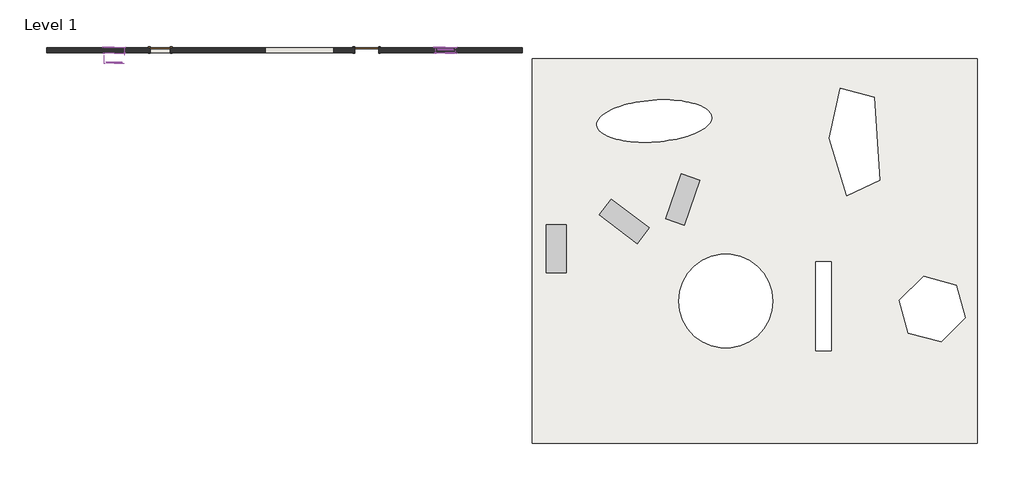
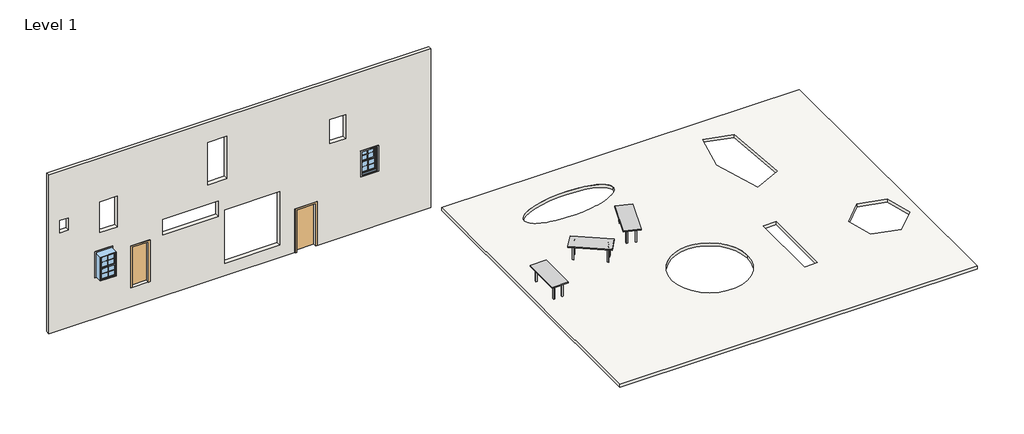
# One storey: 8 proxies, 3 furniture elements, 2 doors, 2 windows, 1 slab, 1 wall.
"""IFC4 building model written with IfcOpenShell, lengths in millimetres."""

import ifcopenshell
import ifcopenshell.guid

model = None  # the IFC model being written
_history = None  # IfcOwnerHistory: only IFC2X3 demands one
_inside = {}  # id of a spatial element -> (the spatial element, [elements in it])
_under = {}  # id of a project, library or spatial element -> (it, [spatial elements below it])
_declared = {}  # id of a project -> (the project, [libraries it declares])
_typed = {}  # id of a type object -> (the type object, [elements of that type])
_made_of = {}  # id of a material, layer set ... -> (it, [elements and type objects made of it])


def new_model(schema):
    """Start an empty IFC model of exactly this schema.

    Asked for "IFC4X3", IfcOpenShell would pick the latest addendum, in which some entities
    have other attributes; the version numbers below select the first issue.
    IFC2X3 requires an IfcOwnerHistory on every rooted entity: one is made here for all.
    """
    global model, _history
    if schema == "IFC4X3":
        model = ifcopenshell.file(schema_version=(4, 3, 0, 0))
    else:
        model = ifcopenshell.file(schema=schema)
    _inside.clear()
    _under.clear()
    _declared.clear()
    _typed.clear()
    _made_of.clear()
    _history = None
    if model.schema == "IFC2X3":
        org = make("IfcOrganization", Name="unknown")
        user = make(
            "IfcPersonAndOrganization",
            ThePerson=make("IfcPerson", FamilyName="unknown"),
            TheOrganization=org,
        )
        app = make(
            "IfcApplication",
            ApplicationDeveloper=org,
            Version="unknown",
            ApplicationFullName="unknown",
            ApplicationIdentifier="unknown",
        )
        _history = make(
            "IfcOwnerHistory",
            OwningUser=user,
            OwningApplication=app,
            ChangeAction="ADDED",
            CreationDate=0,
        )
    return model


def make(cls, **values):
    """One entity of the class cls with the attributes given. An attribute that is None is left unset."""
    return model.create_entity(
        cls, **{name: value for name, value in values.items() if value is not None}
    )


def rooted(cls, **values):
    """An entity with a GlobalId (a new one), such as an element, a storey or a relation."""
    return make(cls, GlobalId=ifcopenshell.guid.new(), OwnerHistory=_history, **values)


def si_unit(unit_type, name, prefix=None):
    """IfcSIUnit, for example si_unit("LENGTHUNIT", "METRE", prefix="MILLI")."""
    return make("IfcSIUnit", UnitType=unit_type, Prefix=prefix, Name=name)


def assignment(units):
    """IfcUnitAssignment: the units of a project."""
    return None if units is None else make("IfcUnitAssignment", Units=units)


def point(xyz):
    """IfcCartesianPoint."""
    return None if xyz is None else make("IfcCartesianPoint", Coordinates=xyz)


def direction(xyz):
    """IfcDirection."""
    return None if xyz is None else make("IfcDirection", DirectionRatios=xyz)


def frame(location, z_axis=None, x_axis=None):
    """IfcAxis2Placement3D, a coordinate frame: its origin and axes. An axis left out is left unset."""
    return make(
        "IfcAxis2Placement3D",
        Location=point(location),
        Axis=direction(z_axis),
        RefDirection=direction(x_axis),
    )


def origin():
    """The frame at (0, 0, 0) with its axes left unset."""
    return frame((0.0, 0.0, 0.0))


def origin_with_axes():
    """The frame at (0, 0, 0) with the z axis (0, 0, 1) and the x axis (1, 0, 0) written out."""
    return frame((0.0, 0.0, 0.0), z_axis=(0.0, 0.0, 1.0), x_axis=(1.0, 0.0, 0.0))


def place(relative_to, where):
    """IfcLocalPlacement: puts the frame where relative to a parent placement (None: the world)."""
    return make(
        "IfcLocalPlacement", PlacementRelTo=relative_to, RelativePlacement=where
    )


def context(
    kind, dimensions, precision=None, world=None, true_north=None, identifier=None
):
    """IfcGeometricRepresentationContext, for example the 3D "Model" context."""
    return make(
        "IfcGeometricRepresentationContext",
        ContextIdentifier=identifier,
        ContextType=kind,
        CoordinateSpaceDimension=dimensions,
        Precision=precision,
        WorldCoordinateSystem=world,
        TrueNorth=true_north,
    )


def project(units=None, contexts=None):
    """IfcProject with its units and contexts."""
    return rooted(
        "IfcProject",
        Name="project",
        RepresentationContexts=contexts,
        UnitsInContext=assignment(units),
    )


def spatial(cls, under=None, at=None, **own):
    """A site, building, storey or space (cls), placed at a placement, below another one or the project."""
    s = rooted(cls, ObjectPlacement=at, **own)
    if under is not None:
        _under.setdefault(under.id(), (under, []))[1].append(s)
    return s


def polyline(points):
    """IfcPolyline through the points."""
    return make("IfcPolyline", Points=[point(p) for p in points])


def circle_curve(where, radius):
    """IfcCircle in the frame where."""
    return make("IfcCircle", Position=where, Radius=radius)


def ellipse_curve(where, semi_axis1, semi_axis2):
    """IfcEllipse in the frame where."""
    return make(
        "IfcEllipse", Position=where, SemiAxis1=semi_axis1, SemiAxis2=semi_axis2
    )


def trimmed(basis, trim1, trim2, sense, master):
    """IfcTrimmedCurve: the piece of a basis curve between two trims."""
    return make(
        "IfcTrimmedCurve",
        BasisCurve=basis,
        Trim1=trim1,
        Trim2=trim2,
        SenseAgreement=sense,
        MasterRepresentation=master,
    )


def outline(outer, holes=None, kind="AREA"):
    """IfcArbitraryClosedProfileDef: a profile drawn as a closed curve; with holes, ...WithVoids."""
    if holes is None:
        return make("IfcArbitraryClosedProfileDef", ProfileType=kind, OuterCurve=outer)
    return make(
        "IfcArbitraryProfileDefWithVoids",
        ProfileType=kind,
        OuterCurve=outer,
        InnerCurves=holes,
    )


def extrude(swept, where, along, depth):
    """IfcExtrudedAreaSolid: the profile swept, set in the frame where, extruded along a direction by depth."""
    return make(
        "IfcExtrudedAreaSolid",
        SweptArea=swept,
        Position=where,
        ExtrudedDirection=direction(along),
        Depth=depth,
    )


def shape(context_of_items, identifier, shape_type, items):
    """IfcShapeRepresentation: the items that make up one representation, for example the "Body"."""
    return make(
        "IfcShapeRepresentation",
        ContextOfItems=context_of_items,
        RepresentationIdentifier=identifier,
        RepresentationType=shape_type,
        Items=items,
    )


def source(mapping_origin, context_of_items, identifier, shape_type, items):
    """IfcRepresentationMap: a shape defined once, which mapped items show again and again."""
    return make(
        "IfcRepresentationMap",
        MappingOrigin=mapping_origin,
        MappedRepresentation=shape(context_of_items, identifier, shape_type, items),
    )


def transform(
    local_origin,
    x_axis=None,
    y_axis=None,
    z_axis=None,
    scale=None,
    scale2=None,
    scale3=None,
    uniform=True,
):
    """IfcCartesianTransformationOperator3D, or its non-uniform kind. x_axis, y_axis, z_axis: its Axis1, 2, 3."""
    if uniform:
        return make(
            "IfcCartesianTransformationOperator3D",
            Axis1=direction(x_axis),
            Axis2=direction(y_axis),
            LocalOrigin=point(local_origin),
            Scale=scale,
            Axis3=direction(z_axis),
        )
    return make(
        "IfcCartesianTransformationOperator3DnonUniform",
        Axis1=direction(x_axis),
        Axis2=direction(y_axis),
        LocalOrigin=point(local_origin),
        Scale=scale,
        Axis3=direction(z_axis),
        Scale2=scale2,
        Scale3=scale3,
    )


def mapped(mapping_source, mapping_target):
    """IfcMappedItem: shows the shape of a source again, moved by a transform."""
    return make(
        "IfcMappedItem", MappingSource=mapping_source, MappingTarget=mapping_target
    )


def made_of(thing, what):
    """Note that an element or type object is made of a material, layer set ...; save() writes the relation."""
    if what is not None:
        _made_of.setdefault(what.id(), (what, []))[1].append(thing)
    return thing


def element(
    cls,
    number,
    at=None,
    inside=None,
    cuts=None,
    type_object=None,
    material=None,
    context=None,
    identifier="Body",
    shape_type=None,
    held_by="IfcProductDefinitionShape",
    body=None,
    shapes=None,
    **own,
):
    """One element of the class cls, such as IfcWall. Its Tag is "e" and its number.

    at: its placement. inside: the storey or other place that contains it. cuts: it is an
    opening in that element (IfcRelVoidsElement). A single representation is given by context,
    identifier, shape_type and body (its items); several are given by shapes. held_by: the class
    of the entity that holds the representations. save() writes the other relations.
    """
    e = rooted(cls, Tag="e%d" % number, ObjectPlacement=at, **own)
    if body is not None:
        shapes = [shape(context, identifier, shape_type, body)]
    if shapes is not None:
        e.Representation = make(held_by, Representations=shapes)
    if inside is not None:
        _inside.setdefault(inside.id(), (inside, []))[1].append(e)
    if cuts is not None:
        rooted(
            "IfcRelVoidsElement", RelatingBuildingElement=cuts, RelatedOpeningElement=e
        )
    if type_object is not None:
        _typed.setdefault(type_object.id(), (type_object, []))[1].append(e)
    return made_of(e, material)


def aggregate(whole, parts):
    """IfcRelAggregates: a whole, such as a stair, and the parts it consists of."""
    return rooted("IfcRelAggregates", RelatingObject=whole, RelatedObjects=parts)


def save(model, path):
    """Write the relations noted so far, then the file.

    IfcRelAggregates (storeys below a building ...), IfcRelContainedInSpatialStructure (elements
    in a storey), IfcRelDefinesByType, IfcRelAssociatesMaterial and IfcRelDeclares: one each for
    every whole, place, type object, material and project.
    """
    for whole, parts in _under.values():
        aggregate(whole, parts)
    for where, things in _inside.values():
        rooted(
            "IfcRelContainedInSpatialStructure",
            RelatedElements=things,
            RelatingStructure=where,
        )
    for kind, things in _typed.values():
        rooted("IfcRelDefinesByType", RelatedObjects=things, RelatingType=kind)
    for what, things in _made_of.values():
        rooted("IfcRelAssociatesMaterial", RelatedObjects=things, RelatingMaterial=what)
    for by, libraries in _declared.values():
        rooted("IfcRelDeclares", RelatingContext=by, RelatedDefinitions=libraries)
    model.write(path)


def plane_surface(at):
    """IfcPlane: the flat surface through the origin of the frame at, square to its z axis."""
    return make("IfcPlane", Position=at)


def revolved_surface(curve, axis_point, axis_direction):
    """IfcSurfaceOfRevolution: the curve turned about the line through axis_point along axis_direction."""
    return make(
        "IfcSurfaceOfRevolution",
        SweptCurve=make("IfcArbitraryOpenProfileDef", ProfileType="CURVE", Curve=curve),
        AxisPosition=make("IfcAxis1Placement", Location=point(axis_point), Axis=direction(axis_direction)),
    )


def extruded_surface(curve, direction_of_extrusion, depth):
    """IfcSurfaceOfLinearExtrusion: the curve pushed along a direction by depth."""
    return make(
        "IfcSurfaceOfLinearExtrusion",
        SweptCurve=make("IfcArbitraryOpenProfileDef", ProfileType="CURVE", Curve=curve),
        ExtrudedDirection=direction(direction_of_extrusion),
        Depth=depth,
    )


def advanced_brep(points, edges, surfaces, faces):
    """IfcAdvancedBrep: a solid bounded by faces that lie on surfaces and meet in shared edges.

    An edge is (start, end): straight between two places in points (the first is 0);
    or (start, end, curve); or (start, end, curve, False) where it runs against its curve.
    A face is (place in surfaces, loops), or (place, loops, False) where it looks against
    its surface's normal. A loop lists edges by number (the first is 1), with a minus sign
    where the edge is run from its end to its start. The first loop is the outer one.
    """
    corners = [point(p) for p in points]
    vertices = [make("IfcVertexPoint", VertexGeometry=c) for c in corners]
    made = []
    for start, end, *more in edges:
        made.append(
            make(
                "IfcEdgeCurve",
                EdgeStart=vertices[start],
                EdgeEnd=vertices[end],
                EdgeGeometry=more[0] if more else make("IfcPolyline", Points=[corners[start], corners[end]]),
                SameSense=more[1] if len(more) > 1 else True,
            )
        )
    hull = []
    for where, loops, *sense in faces:
        bounds = []
        for j, loop in enumerate(loops):
            ring = [make("IfcOrientedEdge", EdgeElement=made[abs(k) - 1], Orientation=k > 0) for k in loop]
            bounds.append(
                make(
                    "IfcFaceOuterBound" if j == 0 else "IfcFaceBound",
                    Bound=make("IfcEdgeLoop", EdgeList=ring),
                    Orientation=True,
                )
            )
        hull.append(make("IfcAdvancedFace", Bounds=bounds, FaceSurface=surfaces[where], SameSense=sense[0] if sense else True))
    return make("IfcAdvancedBrep", Outer=make("IfcClosedShell", CfsFaces=hull))


def m_muntin_pattern_2x2_m_muntin_pattern_2x2_aaec3afb(model_context):
    return source(origin(), model_context, "Body", "SweptSolid", [
        extrude(outline(polyline([(257.1375, -6.35), (257.1375, -298.8), (244.4375, -298.8), (244.4375, -6.35), (0.0, -6.35), (0.0, 6.35), (244.4375, 6.35), (244.4375, 298.8), (257.1375, 298.8), (257.1375, 6.35), (501.575, 6.35), (501.575, -6.35), (257.1375, -6.35)])), frame((0.0, 9.525, 0.0), z_axis=(0.0, 1.0, 0.0), x_axis=(0.0, 0.0, 1.0)), (0.0, 0.0, 1.0), 12.7),
        extrude(outline(polyline([(257.1375, -6.35), (257.1375, -298.8), (244.4375, -298.8), (244.4375, -6.35), (0.0, -6.35), (0.0, 6.35), (244.4375, 6.35), (244.4375, 298.8), (257.1375, 298.8), (257.1375, 6.35), (501.575, 6.35), (501.575, -6.35), (257.1375, -6.35)])), frame((0.0, -22.225, 0.0), z_axis=(0.0, 1.0, 0.0), x_axis=(0.0, 0.0, 1.0)), (0.0, 0.0, 1.0), 12.7),
    ])


def m_trim_window_exterior_flat_with_sill_e7ff6350(model_context):
    return source(origin(), model_context, "Body", "SweptSolid", [
        extrude(outline(polyline([(435.0, -1220.4323709), (435.0, -1280.4323709), (-435.0, -1280.4323709), (-435.0, -1220.4323709), (435.0, -1220.4323709)])), origin_with_axes(), (0.0, 0.0, 1.0), 19.05),
        extrude(outline(polyline([(-1230.0, 38.1), (-1202.4580645, 38.1), (-1200.0, 19.05), (-1200.0, 0.0), (-1220.4323709, 0.0), (-1220.4323709, 19.05), (-1230.0, 19.05), (-1230.0, 38.1)])), frame((-447.7, 0.0, 0.0), z_axis=(1.0, 0.0, 0.0), x_axis=(0.0, 1.0, 0.0)), (0.0, 0.0, 1.0), 895.4),
        extrude(outline(polyline([(-435.0, 60.0), (435.0, 60.0), (435.0, -1200.0), (375.0, -1200.0), (375.0, 0.0), (-375.0, 0.0), (-375.0, -1200.0), (-435.0, -1200.0), (-435.0, 60.0)])), origin_with_axes(), (0.0, 0.0, 1.0), 19.05),
    ])


def m_trim_window_interior_flat_picture_frame_31bd2320(model_context):
    return source(origin(), model_context, "Body", "SweptSolid", [
        extrude(outline(polyline([(422.3, 47.3), (422.3, -1247.3), (-422.3, -1247.3), (-422.3, 47.3), (422.3, 47.3)]), holes=[polyline([(362.3, -12.7), (-362.3, -12.7), (-362.3, -1187.3), (362.3, -1187.3), (362.3, -12.7)])]), origin_with_axes(), (0.0, 0.0, 1.0), 30.0),
    ])


def m_single_flush_0762_x_2032mm_0c256fab(model_context):
    return source(origin(), model_context, "Body", "SweptSolid", [
        extrude(outline(polyline([(2108.0, -457.0), (0.0, -457.0), (0.0, -381.0), (2032.0, -381.0), (2032.0, 381.0), (0.0, 381.0), (0.0, 457.0), (2108.0, 457.0), (2108.0, -457.0)])), frame((0.0, 100.0, 0.0), z_axis=(0.0, 1.0, 0.0), x_axis=(0.0, 0.0, 1.0)), (0.0, 0.0, 1.0), 25.0),
        extrude(outline(polyline([(2108.0, 457.0), (2108.0, -457.0), (0.0, -457.0), (0.0, -381.0), (2032.0, -381.0), (2032.0, 381.0), (0.0, 381.0), (0.0, 457.0), (2108.0, 457.0)])), frame((0.0, -125.0, 0.0), z_axis=(0.0, 1.0, 0.0), x_axis=(0.0, 0.0, 1.0)), (0.0, 0.0, 1.0), 25.0),
        extrude(outline(polyline([(381.0, 49.0), (-381.0, 49.0), (-381.0, 100.0), (381.0, 100.0), (381.0, 49.0)])), origin_with_axes(), (0.0, 0.0, 1.0), 2032.0),
    ])


def m_single_flush_0915_x_2134mm_727434cd(model_context):
    return source(origin(), model_context, "Body", "SweptSolid", [
        extrude(outline(polyline([(2210.0, -533.5), (0.0, -533.5), (0.0, -457.5), (2134.0, -457.5), (2134.0, 457.5), (0.0, 457.5), (0.0, 533.5), (2210.0, 533.5), (2210.0, -533.5)])), frame((0.0, -125.0, 0.0), z_axis=(0.0, 1.0, 0.0), x_axis=(0.0, 0.0, 1.0)), (0.0, 0.0, 1.0), 25.0),
        extrude(outline(polyline([(2210.0, 533.5), (2210.0, -533.5), (0.0, -533.5), (0.0, -457.5), (2134.0, -457.5), (2134.0, 457.5), (0.0, 457.5), (0.0, 533.5), (2210.0, 533.5)])), frame((0.0, 100.0, 0.0), z_axis=(0.0, 1.0, 0.0), x_axis=(0.0, 0.0, 1.0)), (0.0, 0.0, 1.0), 25.0),
        extrude(outline(polyline([(457.5, -49.0), (457.5, -100.0), (-457.5, -100.0), (-457.5, -49.0), (457.5, -49.0)])), origin_with_axes(), (0.0, 0.0, 1.0), 2134.0),
    ])


def m_table_rectangular_1830_x_0762mm_a0b3b7a0(model_context):
    return source(origin(), model_context, "Body", "SweptSolid", [
        extrude(outline(polyline([(699.1, 190.5), (699.1, 165.1), (-699.1, 165.1), (-699.1, 190.5), (699.1, 190.5)])), frame((0.0, 0.0, 609.6), z_axis=(0.0, 0.0, 1.0), x_axis=(1.0, 0.0, 0.0)), (0.0, 0.0, 1.0), 101.6),
        extrude(outline(polyline([(699.1, -190.5), (-699.1, -190.5), (-699.1, -165.1), (699.1, -165.1), (699.1, -190.5)])), frame((0.0, 0.0, 609.6), z_axis=(0.0, 0.0, 1.0), x_axis=(1.0, 0.0, 0.0)), (0.0, 0.0, 1.0), 101.6),
        extrude(outline(polyline([(-711.8, -165.1), (-737.2, -165.1), (-737.2, 165.1), (-711.8, 165.1), (-711.8, -165.1)])), frame((0.0, 0.0, 609.6), z_axis=(0.0, 0.0, 1.0), x_axis=(1.0, 0.0, 0.0)), (0.0, 0.0, 1.0), 101.6),
        extrude(outline(polyline([(711.8, -165.1), (711.8, 165.1), (737.2, 165.1), (737.2, -165.1), (711.8, -165.1)])), frame((0.0, 0.0, 609.6), z_axis=(0.0, 0.0, 1.0), x_axis=(1.0, 0.0, 0.0)), (0.0, 0.0, 1.0), 101.6),
        extrude(outline(polyline([(915.0, 381.0), (915.0, -381.0), (-915.0, -381.0), (-915.0, 381.0), (915.0, 381.0)])), frame((0.0, 0.0, 711.2), z_axis=(0.0, 0.0, 1.0), x_axis=(1.0, 0.0, 0.0)), (0.0, 0.0, 1.0), 50.8),
        extrude(outline(polyline([(-699.1, 228.6), (-699.1, 165.1), (-762.6, 165.1), (-762.6, 228.6), (-699.1, 228.6)])), origin_with_axes(), (0.0, 0.0, 1.0), 711.2),
        extrude(outline(polyline([(699.1, 228.6), (762.6, 228.6), (762.6, 165.1), (699.1, 165.1), (699.1, 228.6)])), origin_with_axes(), (0.0, 0.0, 1.0), 711.2),
        extrude(outline(polyline([(-699.1, -228.6), (-762.6, -228.6), (-762.6, -165.1), (-699.1, -165.1), (-699.1, -228.6)])), origin_with_axes(), (0.0, 0.0, 1.0), 711.2),
        extrude(outline(polyline([(699.1, -228.6), (699.1, -165.1), (762.6, -165.1), (762.6, -228.6), (699.1, -228.6)])), origin_with_axes(), (0.0, 0.0, 1.0), 711.2),
    ])


def m_window_double_hung_750_x_1200mm_e21ea802(model_context):
    return source(origin(), model_context, "Body", "SweptSolid", [
        extrude(outline(polyline([(298.8, -469.85), (298.8, -476.2), (-298.8, -476.2), (-298.8, -469.85), (298.8, -469.85)])), frame((0.0, 0.0, 990.6), z_axis=(0.0, 0.0, 1.0), x_axis=(1.0, 0.0, 0.0)), (0.0, 0.0, 1.0), 501.575),
        extrude(outline(polyline([(-298.8, -482.55), (298.8, -482.55), (298.8, -488.9), (-298.8, -488.9), (-298.8, -482.55)])), frame((0.0, 0.0, 990.6), z_axis=(0.0, 0.0, 1.0), x_axis=(1.0, 0.0, 0.0)), (0.0, 0.0, 1.0), 501.575),
        extrude(outline(polyline([(298.8, -425.4), (298.8, -431.75), (-298.8, -431.75), (-298.8, -425.4), (298.8, -425.4)])), frame((0.0, 0.0, 1536.625), z_axis=(0.0, 0.0, 1.0), x_axis=(1.0, 0.0, 0.0)), (0.0, 0.0, 1.0), 501.575),
        extrude(outline(polyline([(-298.8, -438.1), (298.8, -438.1), (298.8, -444.45), (-298.8, -444.45), (-298.8, -438.1)])), frame((0.0, 0.0, 1536.625), z_axis=(0.0, 0.0, 1.0), x_axis=(1.0, 0.0, 0.0)), (0.0, 0.0, 1.0), 501.575),
        extrude(outline(polyline([(1536.625, -343.25), (946.15, -343.25), (946.15, 343.25), (1536.625, 343.25), (1536.625, -343.25)]), holes=[polyline([(1492.175, 298.8), (990.6, 298.8), (990.6, -298.8), (1492.175, -298.8), (1492.175, 298.8)])]), frame((0.0, -501.6, 0.0), z_axis=(0.0, 1.0, 0.0), x_axis=(0.0, 0.0, 1.0)), (0.0, 0.0, 1.0), 44.45),
        extrude(outline(polyline([(2082.65, -343.25), (1492.175, -343.25), (1492.175, 343.25), (2082.65, 343.25), (2082.65, -343.25)]), holes=[polyline([(2038.2, 298.8), (1536.625, 298.8), (1536.625, -298.8), (2038.2, -298.8), (2038.2, 298.8)])]), frame((0.0, -457.15, 0.0), z_axis=(0.0, 1.0, 0.0), x_axis=(0.0, 0.0, 1.0)), (0.0, 0.0, 1.0), 44.45),
        extrude(outline(polyline([(2114.4, -375.0), (914.4, -375.0), (914.4, 375.0), (2114.4, 375.0), (2114.4, -375.0)]), holes=[polyline([(2082.65, 343.25), (946.15, 343.25), (946.15, -343.25), (2082.65, -343.25), (2082.65, 343.25)])]), frame((0.0, -514.3, 0.0), z_axis=(0.0, 1.0, 0.0), x_axis=(0.0, 0.0, 1.0)), (0.0, 0.0, 1.0), 633.35),
    ])


def m_window_double_hung_750_x_1200mm_41070976(model_context):
    return source(origin(), model_context, "Body", "SweptSolid", [
        extrude(outline(polyline([(298.8, 30.15), (298.8, 23.8), (-298.8, 23.8), (-298.8, 30.15), (298.8, 30.15)])), frame((0.0, 0.0, 990.6), z_axis=(0.0, 0.0, 1.0), x_axis=(1.0, 0.0, 0.0)), (0.0, 0.0, 1.0), 501.575),
        extrude(outline(polyline([(-298.8, 17.45), (298.8, 17.45), (298.8, 11.1), (-298.8, 11.1), (-298.8, 17.45)])), frame((0.0, 0.0, 990.6), z_axis=(0.0, 0.0, 1.0), x_axis=(1.0, 0.0, 0.0)), (0.0, 0.0, 1.0), 501.575),
        extrude(outline(polyline([(298.8, 74.6), (298.8, 68.25), (-298.8, 68.25), (-298.8, 74.6), (298.8, 74.6)])), frame((0.0, 0.0, 1536.625), z_axis=(0.0, 0.0, 1.0), x_axis=(1.0, 0.0, 0.0)), (0.0, 0.0, 1.0), 501.575),
        extrude(outline(polyline([(-298.8, 61.9), (298.8, 61.9), (298.8, 55.55), (-298.8, 55.55), (-298.8, 61.9)])), frame((0.0, 0.0, 1536.625), z_axis=(0.0, 0.0, 1.0), x_axis=(1.0, 0.0, 0.0)), (0.0, 0.0, 1.0), 501.575),
        extrude(outline(polyline([(1536.625, -343.25), (946.15, -343.25), (946.15, 343.25), (1536.625, 343.25), (1536.625, -343.25)]), holes=[polyline([(1492.175, 298.8), (990.6, 298.8), (990.6, -298.8), (1492.175, -298.8), (1492.175, 298.8)])]), frame((0.0, -1.6, 0.0), z_axis=(0.0, 1.0, 0.0), x_axis=(0.0, 0.0, 1.0)), (0.0, 0.0, 1.0), 44.45),
        extrude(outline(polyline([(2082.65, -343.25), (1492.175, -343.25), (1492.175, 343.25), (2082.65, 343.25), (2082.65, -343.25)]), holes=[polyline([(2038.2, 298.8), (1536.625, 298.8), (1536.625, -298.8), (2038.2, -298.8), (2038.2, 298.8)])]), frame((0.0, 42.85, 0.0), z_axis=(0.0, 1.0, 0.0), x_axis=(0.0, 0.0, 1.0)), (0.0, 0.0, 1.0), 44.45),
        extrude(outline(polyline([(2114.4, -375.0), (914.4, -375.0), (914.4, 375.0), (2114.4, 375.0), (2114.4, -375.0)]), holes=[polyline([(2082.65, 343.25), (946.15, 343.25), (946.15, -343.25), (2082.65, -343.25), (2082.65, 343.25)])]), frame((0.0, -14.3, 0.0), z_axis=(0.0, 1.0, 0.0), x_axis=(0.0, 0.0, 1.0)), (0.0, 0.0, 1.0), 133.35),
        extrude(outline(polyline([(2114.4, 375.0), (2114.4, -375.0), (914.4, -375.0), (914.4, 375.0), (2114.4, 375.0)]), holes=[polyline([(2095.35, 355.95), (933.45, 355.95), (933.45, -355.95), (2095.35, -355.95), (2095.35, 355.95)])]), frame((0.0, -100.0, 0.0), z_axis=(0.0, 1.0, 0.0), x_axis=(0.0, 0.0, 1.0)), (0.0, 0.0, 1.0), 85.7),
    ])


model = new_model("IFC4")

# Units and contexts
model_context = context("Model", 3, world=origin())
ifc_project = project(units=[si_unit("LENGTHUNIT", "METRE", prefix="MILLI")], contexts=[model_context])

# Site, building, storey
site = spatial("IfcSite", under=ifc_project)
building = spatial("IfcBuilding", under=site)
storey = spatial("IfcBuildingStorey", under=building, Name="Level 1", Elevation=0.0)

# Proxies
placement = place(None, origin())
m_muntin_pattern_2x2_m_muntin_pattern_2x2_shape = m_muntin_pattern_2x2_m_muntin_pattern_2x2_aaec3afb(model_context)
element("IfcBuildingElementProxy", 1, Name="M_Muntin Pattern_2x2 : M_Muntin Pattern_2x2", ObjectType="M_Muntin Pattern_2x2 : M_Muntin Pattern_2x2", at=placement, inside=storey, context=model_context, shape_type="MappedRepresentation", body=[
    mapped(m_muntin_pattern_2x2_m_muntin_pattern_2x2_shape, transform((-13755.2543844, 2099.5505832, 3404.9440493), x_axis=(1.0, 0.0, 0.0), y_axis=(0.0, 1.0, 0.0), z_axis=(0.0, 0.0, 1.0))),
])
element("IfcBuildingElementProxy", 2, Name="M_Muntin Pattern_2x2 : M_Muntin Pattern_2x2", ObjectType="M_Muntin Pattern_2x2 : M_Muntin Pattern_2x2", at=placement, inside=storey, context=model_context, shape_type="MappedRepresentation", body=[
    mapped(m_muntin_pattern_2x2_m_muntin_pattern_2x2_shape, transform((-13755.2543844, 2055.1005832, 2858.9190493), x_axis=(1.0, 0.0, 0.0), y_axis=(0.0, 1.0, 0.0), z_axis=(0.0, 0.0, 1.0))),
])
element("IfcBuildingElementProxy", 3, Name="M_Muntin Pattern_2x2 : M_Muntin Pattern_2x2", ObjectType="M_Muntin Pattern_2x2 : M_Muntin Pattern_2x2", at=placement, inside=storey, context=model_context, shape_type="MappedRepresentation", body=[
    mapped(m_muntin_pattern_2x2_m_muntin_pattern_2x2_shape, transform((-26427.6862127, 1599.5505832, 2762.3712435), x_axis=(1.0, 0.0, 0.0), y_axis=(0.0, 1.0, 0.0), z_axis=(0.0, 0.0, 1.0))),
])
element("IfcBuildingElementProxy", 4, Name="M_Muntin Pattern_2x2 : M_Muntin Pattern_2x2", ObjectType="M_Muntin Pattern_2x2 : M_Muntin Pattern_2x2", at=placement, inside=storey, context=model_context, shape_type="MappedRepresentation", body=[
    mapped(m_muntin_pattern_2x2_m_muntin_pattern_2x2_shape, transform((-26427.6862127, 1555.1005832, 2216.3462435), x_axis=(1.0, 0.0, 0.0), y_axis=(0.0, 1.0, 0.0), z_axis=(0.0, 0.0, 1.0))),
])
m_trim_window_exterior_flat_with_sill_shape = m_trim_window_exterior_flat_with_sill_e7ff6350(model_context)
element("IfcBuildingElementProxy", 5, Name="M_Trim-Window-Exterior-Flat : with Sill", ObjectType="M_Trim-Window-Exterior-Flat : with Sill", at=placement, inside=storey, context=model_context, shape_type="MappedRepresentation", body=[
    mapped(m_trim_window_exterior_flat_with_sill_shape, transform((-13755.2543844, 2134.4755832, 3982.7190493), x_axis=(-1.0, 0.0, 0.0), y_axis=(0.0, 0.0, 1.0), z_axis=(0.0, 1.0, 0.0))),
])
element("IfcBuildingElementProxy", 6, Name="M_Trim-Window-Exterior-Flat : with Sill", ObjectType="M_Trim-Window-Exterior-Flat : with Sill", at=placement, inside=storey, context=model_context, shape_type="MappedRepresentation", body=[
    mapped(m_trim_window_exterior_flat_with_sill_shape, transform((-26427.6862127, 2134.4755832, 3340.1462435), x_axis=(-1.0, 0.0, 0.0), y_axis=(0.0, 0.0, 1.0), z_axis=(0.0, 1.0, 0.0))),
])
m_trim_window_interior_flat_picture_frame_shape = m_trim_window_interior_flat_picture_frame_31bd2320(model_context)
element("IfcBuildingElementProxy", 7, Name="M_Trim-Window-Interior-Flat : Picture Frame", ObjectType="M_Trim-Window-Interior-Flat : Picture Frame", at=placement, inside=storey, context=model_context, shape_type="MappedRepresentation", body=[
    mapped(m_trim_window_interior_flat_picture_frame_shape, transform((-13755.2543844, 1934.4755832, 3982.7190493), x_axis=(1.0, 0.0, 0.0), y_axis=(0.0, 0.0, 1.0), z_axis=(0.0, -1.0, 0.0))),
])
element("IfcBuildingElementProxy", 8, Name="M_Trim-Window-Interior-Flat : Picture Frame", ObjectType="M_Trim-Window-Interior-Flat : Picture Frame", at=placement, inside=storey, context=model_context, shape_type="MappedRepresentation", body=[
    mapped(m_trim_window_interior_flat_picture_frame_shape, transform((-26427.6862127, 1934.4755832, 3340.1462435), x_axis=(1.0, 0.0, 0.0), y_axis=(0.0, 0.0, 1.0), z_axis=(0.0, -1.0, 0.0))),
])

# Doors
m_single_flush_0762_x_2032mm_shape = m_single_flush_0762_x_2032mm_0c256fab(model_context)
element("IfcDoor", 9, ObjectType="M_Single-Flush : 0762 x 2032mm", at=placement, inside=storey, context=model_context, shape_type="MappedRepresentation", body=[
    mapped(m_single_flush_0762_x_2032mm_shape, transform((-24671.6862127, 2034.4755832, 968.0), x_axis=(1.0, 0.0, 0.0), y_axis=(0.0, 1.0, 0.0), z_axis=(0.0, 0.0, 1.0))),
])
m_single_flush_0915_x_2134mm_shape = m_single_flush_0915_x_2134mm_727434cd(model_context)
element("IfcDoor", 10, ObjectType="M_Single-Flush : 0915 x 2134mm", at=placement, inside=storey, context=model_context, shape_type="MappedRepresentation", body=[
    mapped(m_single_flush_0915_x_2134mm_shape, transform((-16774.8897659, 2034.4755832, 0.0), x_axis=(-1.0, 0.0, 0.0), y_axis=(0.0, -1.0, 0.0), z_axis=(0.0, 0.0, 1.0))),
])

# Furniture
m_table_rectangular_1830_x_0762mm_shape = m_table_rectangular_1830_x_0762mm_a0b3b7a0(model_context)
element("IfcFurniture", 11, ObjectType="M_Table-Rectangular : 1830 x 0762mm", at=placement, inside=storey, context=model_context, shape_type="MappedRepresentation", body=[
    mapped(m_table_rectangular_1830_x_0762mm_shape, transform((-4676.3852744, -3681.7142207, 0.0), x_axis=(-0.32556815445715137, -0.9455185755993186, 0.0), y_axis=(0.9455185755993186, -0.32556815445715137, 0.0), z_axis=(0.0, 0.0, 1.0))),
])
element("IfcFurniture", 12, ObjectType="M_Table-Rectangular : 1830 x 0762mm", at=placement, inside=storey, context=model_context, shape_type="MappedRepresentation", body=[
    mapped(m_table_rectangular_1830_x_0762mm_shape, transform((-6912.0232604, -4514.409007, 0.0), x_axis=(0.7986355100472892, -0.601815023152053, 0.0), y_axis=(0.601815023152053, 0.7986355100472892, 0.0), z_axis=(0.0, 0.0, 1.0))),
])
element("IfcFurniture", 13, ObjectType="M_Table-Rectangular : 1830 x 0762mm", at=placement, inside=storey, context=model_context, shape_type="MappedRepresentation", body=[
    mapped(m_table_rectangular_1830_x_0762mm_shape, transform((-9517.3897659, -5565.5244168, 0.0), x_axis=(0.0, 1.0, 0.0), y_axis=(-1.0, 0.0, 0.0), z_axis=(0.0, 0.0, 1.0))),
])

# Slab
element("IfcSlab", 14, ObjectType="Generic 150mm", at=placement, inside=storey, context=model_context, shape_type="AdvancedBrep", body=[
    advanced_brep(
    [(-10438.0920872, 1704.9536342, -150.0), (6597.1361468, 1704.9536342, -150.0), (6597.1361468, -12995.0463658, -150.0), (-10438.0920872, -12995.0463658, -150.0), (402.6850474, -6063.7932352, -150.0), (402.6850474, -9463.7932352, -150.0), (1002.6850474, -9463.7932352, -150.0), (1002.6850474, -6063.7932352, -150.0), (-1226.5132944, -7566.8871411, -150.0), (-4826.5132944, -7566.8871411, -150.0), (3950.2905395, -8793.2666419, -150.0), (5205.9941136, -9129.7314005, -150.0), (6125.2329292, -8210.492585, -150.0), (5788.7681706, -6954.7890108, -150.0), (4533.0645964, -6618.3242522, -150.0), (3613.8257808, -7537.5630677, -150.0), (2640.3105602, 236.4658339, -150.0), (1342.8691088, 584.1142231, -150.0), (924.6812259, -1326.1660948, -150.0), (1597.1361468, -3525.6670335, -150.0), (2862.1361468, -2935.7878459, -150.0), (-3571.6563241, -523.7317463, -150.0), (-7960.9381452, -830.6602307, -150.0), (6597.1361468, 1704.9536342, 0.0), (-10438.0920872, 1704.9536342, 0.0), (-10438.0920872, -12995.0463658, 0.0), (6597.1361468, -12995.0463658, 0.0), (402.6850474, -9463.7932352, 0.0), (402.6850474, -6063.7932352, 0.0), (1002.6850474, -6063.7932352, 0.0), (1002.6850474, -9463.7932352, 0.0), (-4826.5132944, -7566.8871411, 0.0), (-1226.5132944, -7566.8871411, 0.0), (5205.9941136, -9129.7314005, 0.0), (3950.2905395, -8793.2666419, 0.0), (3613.8257808, -7537.5630677, 0.0), (4533.0645964, -6618.3242522, 0.0), (5788.7681706, -6954.7890108, 0.0), (6125.2329292, -8210.492585, 0.0), (1342.8691088, 584.1142231, 0.0), (2640.3105602, 236.4658339, 0.0), (2862.1361468, -2935.7878459, 0.0), (1597.1361468, -3525.6670335, 0.0), (924.6812259, -1326.1660948, 0.0), (-7960.9381452, -830.6602307, 0.0), (-3571.6563241, -523.7317463, 0.0)],
    [
        (0, 1),
        (1, 2),
        (2, 3),
        (3, 0),
        (4, 5),
        (5, 6),
        (6, 7),
        (7, 4),
        (8, 9, circle_curve(frame((-3026.5132944, -7566.8871411, -150.0), z_axis=(0.0, 0.0, 1.0), x_axis=(-1.0, 0.0, 0.0)), 1800.0)),
        (9, 8, circle_curve(frame((-3026.5132944, -7566.8871411, -150.0), z_axis=(0.0, 0.0, 1.0), x_axis=(-1.0, 0.0, 0.0)), 1800.0)),
        (10, 11),
        (11, 12),
        (12, 13),
        (13, 14),
        (14, 15),
        (15, 10),
        (16, 17),
        (17, 18),
        (18, 19),
        (19, 20),
        (20, 16),
        (21, 22, ellipse_curve(frame((-5766.2972347, -677.1959885, -150.0), z_axis=(0.0, 0.0, 1.0), x_axis=(-0.9975640502598249, -0.06975647374411696, 0.0)), 2200.0, 800.0)),
        (22, 21, ellipse_curve(frame((-5766.2972347, -677.1959885, -150.0), z_axis=(0.0, 0.0, 1.0), x_axis=(-0.9975640502598249, -0.06975647374411696, 0.0)), 2200.0, 800.0)),
        (23, 24),
        (24, 25),
        (25, 26),
        (26, 23),
        (27, 28),
        (28, 29),
        (29, 30),
        (30, 27),
        (31, 32, circle_curve(frame((-3026.5132944, -7566.8871411, 0.0), z_axis=(0.0, 0.0, -1.0), x_axis=(-1.0, 0.0, 0.0)), 1800.0)),
        (32, 31, circle_curve(frame((-3026.5132944, -7566.8871411, 0.0), z_axis=(0.0, 0.0, -1.0), x_axis=(-1.0, 0.0, 0.0)), 1800.0)),
        (33, 34),
        (34, 35),
        (35, 36),
        (36, 37),
        (37, 38),
        (38, 33),
        (39, 40),
        (40, 41),
        (41, 42),
        (42, 43),
        (43, 39),
        (44, 45, ellipse_curve(frame((-5766.2972347, -677.1959885, 0.0), z_axis=(0.0, 0.0, -1.0), x_axis=(-0.9975640502598249, -0.06975647374411696, 0.0)), 2200.0, 800.0)),
        (45, 44, ellipse_curve(frame((-5766.2972347, -677.1959885, 0.0), z_axis=(0.0, 0.0, -1.0), x_axis=(-0.9975640502598249, -0.06975647374411696, 0.0)), 2200.0, 800.0)),
        (0, 24),
        (23, 1),
        (26, 2),
        (25, 3),
        (4, 28),
        (27, 5),
        (30, 6),
        (29, 7),
        (8, 32),
        (31, 9),
        (10, 34),
        (33, 11),
        (38, 12),
        (37, 13),
        (36, 14),
        (35, 15),
        (16, 40),
        (39, 17),
        (18, 43),
        (42, 19),
        (41, 20),
        (21, 45),
        (44, 22),
    ],
    [
        plane_surface(frame((5561.9079128, 1704.9536342, -150.0), z_axis=(0.0, 0.0, -1.0), x_axis=(1.0, 0.0, 0.0))),
        plane_surface(frame((5561.9079128, 1704.9536342, 0.0), z_axis=(0.0, 0.0, 1.0), x_axis=(-1.0, 0.0, 0.0))),
        plane_surface(frame((-10438.0920872, 1704.9536342, -150.0), z_axis=(0.0, 1.0, 0.0), x_axis=(0.0, 0.0, 1.0))),
        plane_surface(frame((6597.1361468, 1704.9536342, -150.0), z_axis=(1.0, 0.0, 0.0), x_axis=(0.0, 0.0, 1.0))),
        plane_surface(frame((6597.1361468, -12995.0463658, -150.0), z_axis=(0.0, -1.0, 0.0), x_axis=(0.0, 0.0, 1.0))),
        plane_surface(frame((-10438.0920872, -12995.0463658, -150.0), z_axis=(-1.0, 0.0, 0.0), x_axis=(0.0, 0.0, 1.0))),
        plane_surface(frame((402.6850474, -6063.7932352, 754.8), z_axis=(1.0, 0.0, 0.0), x_axis=(0.0, 0.0, -1.0))),
        plane_surface(frame((402.6850474, -9463.7932352, 754.8), z_axis=(0.0, 1.0, 0.0), x_axis=(0.0, 0.0, -1.0))),
        plane_surface(frame((1002.6850474, -9463.7932352, 754.8), z_axis=(-1.0, 0.0, 0.0), x_axis=(0.0, 0.0, -1.0))),
        plane_surface(frame((1002.6850474, -6063.7932352, 754.8), z_axis=(0.0, -1.0, 0.0), x_axis=(0.0, 0.0, -1.0))),
        revolved_surface(polyline([(-4826.5132944, -7566.8871411, 0.0), (-4826.5132944, -7566.8871411, -150.0)]), (-3026.5132944, -7566.8871411, -454.8), (0.0, 0.0, 1.0)),
        plane_surface(frame((3950.2905395, -8793.2666419, 754.8), z_axis=(0.2588190451025399, 0.9659258262890632, 0.0), x_axis=(0.0, 0.0, -1.0))),
        plane_surface(frame((5205.9941136, -9129.7314005, 754.8), z_axis=(-0.7071067811865333, 0.7071067811865619, 0.0), x_axis=(0.0, 0.0, -1.0))),
        plane_surface(frame((6125.2329292, -8210.492585, 754.8), z_axis=(-0.9659258262890744, -0.2588190451024985, 0.0), x_axis=(0.0, 0.0, -1.0))),
        plane_surface(frame((5788.7681706, -6954.7890108, 754.8), z_axis=(-0.25881904510254333, -0.9659258262890623, 0.0), x_axis=(0.0, 0.0, -1.0))),
        plane_surface(frame((4533.0645964, -6618.3242522, 754.8), z_axis=(0.7071067811865306, -0.7071067811865644, 0.0), x_axis=(0.0, 0.0, -1.0))),
        plane_surface(frame((3613.8257808, -7537.5630677, 754.8), z_axis=(0.965925826289073, 0.2588190451025034, 0.0), x_axis=(0.0, 0.0, -1.0))),
        plane_surface(frame((2640.3105602, 236.4658339, -150.0), z_axis=(-0.25881904510253306, -0.9659258262890651, 0.0), x_axis=(0.0, 0.0, 1.0))),
        plane_surface(frame((924.6812259, -1326.1660948, -150.0), z_axis=(0.9563047559630387, 0.29237170472272644, 0.0), x_axis=(0.0, 0.0, 1.0))),
        plane_surface(frame((1597.1361468, -3525.6670335, -150.0), z_axis=(-0.42261826174069067, 0.9063077870366542, 0.0), x_axis=(0.0, 0.0, 1.0))),
        plane_surface(frame((2862.1361468, -2935.7878459, -150.0), z_axis=(-0.997564050259825, -0.06975647374411523, 0.0), x_axis=(0.0, 0.0, 1.0))),
        plane_surface(frame((1342.8691088, 584.1142231, -150.0), z_axis=(0.9768664776736946, -0.21385014565669358, 0.0), x_axis=(0.0, 0.0, 1.0))),
        extruded_surface(trimmed(ellipse_curve(frame((-5766.2972347, -677.1959885, 150.0), z_axis=(0.0, 0.0, 1.0), x_axis=(-0.9975640502598249, -0.06975647374411696, 0.0)), 2200.0, 800.0), [point((-3571.6563241, -523.7317463, 150.0))], [point((-7960.9381452, -830.6602307, 150.0))], True, "CARTESIAN"), (0.0, 0.0, -150.0), 150.0),
        extruded_surface(trimmed(ellipse_curve(frame((-5766.2972347, -677.1959885, 150.0), z_axis=(0.0, 0.0, 1.0), x_axis=(-0.9975640502598249, -0.06975647374411696, 0.0)), 2200.0, 800.0), [point((-7960.9381452, -830.6602307, 150.0))], [point((-3571.6563241, -523.7317463, 150.0))], True, "CARTESIAN"), (0.0, 0.0, -150.0), 150.0),
    ],
    [
        (0, [[1, 2, 3, 4], [5, 6, 7, 8], [9, 10], [11, 12, 13, 14, 15, 16], [17, 18, 19, 20, 21], [22, 23]]),
        (1, [[24, 25, 26, 27], [28, 29, 30, 31], [32, 33], [34, 35, 36, 37, 38, 39], [40, 41, 42, 43, 44], [45, 46]]),
        (2, [[-1, 47, -24, 48]]),
        (3, [[-2, -48, -27, 49]]),
        (4, [[-3, -49, -26, 50]]),
        (5, [[-4, -50, -25, -47]]),
        (6, [[51, -28, 52, -5]]),
        (7, [[-52, -31, 53, -6]]),
        (8, [[-53, -30, 54, -7]]),
        (9, [[-51, -8, -54, -29]]),
        (10, [[55, -32, 56, -9]]),
        (10, [[-55, -10, -56, -33]]),
        (11, [[57, -34, 58, -11]]),
        (12, [[-58, -39, 59, -12]]),
        (13, [[-59, -38, 60, -13]]),
        (14, [[-60, -37, 61, -14]]),
        (15, [[-61, -36, 62, -15]]),
        (16, [[-57, -16, -62, -35]]),
        (17, [[-17, 63, -40, 64]]),
        (18, [[-19, 65, -43, 66]]),
        (19, [[-20, -66, -42, 67]]),
        (20, [[-21, -67, -41, -63]]),
        (21, [[-18, -64, -44, -65]]),
        (22, [[-22, 68, -45, 69]]),
        (23, [[-23, -69, -46, -68]]),
    ],
),
])

# Wall
element("IfcWall", 15, ObjectType="Generic - 200mm", at=placement, inside=storey, context=model_context, shape_type="SweptSolid", body=[
    extrude(outline(polyline([(8000.0, -29017.3897659), (0.0, -29017.3897659), (0.0, -17232.3897659), (2134.0, -17232.3897659), (2134.0, -16317.3897659), (0.0, -16317.3897659), (0.0, -10817.3897659), (8000.0, -10817.3897659), (8000.0, -29017.3897659)]), holes=[polyline([(968.0, -24290.6862127), (968.0, -25052.6862127), (3000.0, -25052.6862127), (3000.0, -24290.6862127), (968.0, -24290.6862127)]), polyline([(4915.0, -28496.5284847), (5525.0, -28496.5284847), (5525.0, -28090.5284847), (4915.0, -28090.5284847), (4915.0, -28496.5284847)]), polyline([(2140.1462435, -26802.6862127), (3340.1462435, -26802.6862127), (3340.1462435, -26052.6862127), (2140.1462435, -26052.6862127), (2140.1462435, -26802.6862127)]), polyline([(2782.7190493, -14130.2543844), (3982.7190493, -14130.2543844), (3982.7190493, -13380.2543844), (2782.7190493, -13380.2543844), (2782.7190493, -14130.2543844)]), polyline([(4914.4, -15639.9853759), (6114.4, -15639.9853759), (6114.4, -14889.9853759), (4914.4, -14889.9853759), (4914.4, -15639.9853759)]), polyline([(4866.0, -20539.9853759), (4866.0, -21454.9853759), (7000.0, -21454.9853759), (7000.0, -20539.9853759), (4866.0, -20539.9853759)]), polyline([(3328.9271244, -20644.8897659), (3328.9271244, -18024.3599995), (634.0, -18024.3599995), (634.0, -20644.8897659), (3328.9271244, -20644.8897659)]), polyline([(3873.453269, -23605.3752389), (3873.453269, -20944.8897659), (3100.0, -20944.8897659), (3100.0, -23605.3752389), (3873.453269, -23605.3752389)]), polyline([(5800.0, -26593.5284847), (5800.0, -25757.3810809), (4260.1064286, -25757.3810809), (4260.1064286, -26593.5284847), (5800.0, -26593.5284847)])]), frame((0.0, 1934.4755832, 0.0), z_axis=(0.0, 1.0, 0.0), x_axis=(0.0, 0.0, 1.0)), (0.0, 0.0, 1.0), 200.0),
])

# Windows
m_window_double_hung_750_x_1200mm_shape = m_window_double_hung_750_x_1200mm_e21ea802(model_context)
element("IfcWindow", 16, ObjectType="M_Window-Double-Hung : 750 x 1200mm", at=placement, inside=storey, context=model_context, shape_type="MappedRepresentation", body=[
    mapped(m_window_double_hung_750_x_1200mm_shape, transform((-26427.6862127, 2034.4755832, 1225.7462435), x_axis=(1.0, 0.0, 0.0), y_axis=(0.0, 1.0, 0.0), z_axis=(0.0, 0.0, 1.0))),
])
m_window_double_hung_750_x_1200mm_2_shape = m_window_double_hung_750_x_1200mm_41070976(model_context)
element("IfcWindow", 17, ObjectType="M_Window-Double-Hung : 750 x 1200mm", at=placement, inside=storey, context=model_context, shape_type="MappedRepresentation", body=[
    mapped(m_window_double_hung_750_x_1200mm_2_shape, transform((-13755.2543844, 2034.4755832, 1868.3190493), x_axis=(1.0, 0.0, 0.0), y_axis=(0.0, 1.0, 0.0), z_axis=(0.0, 0.0, 1.0))),
])

save(model, "model.ifc")

# Revit data of these elements
# Project information
#   Project Issue Date = "Issue Date"
#   Project Status = "Project Status"
#   Client Name = "Owner"
#   Project Address = "Enter address here"
#   Project Name = "Project Name"
#   Project Number = "0001"
# Type "M_Muntin Pattern_2x2 : M_Muntin Pattern_2x2"
#   Width [instance default] = 1200 mm
#   Thickness = 12.7 mm
#   Height [instance default] = 1200 mm
#   Distance = 19.05 mm
#   Interior Material [instance default] = none
#   Exterior Material [instance default] = none
#   Default Elevation = 0
# Type "M_Trim-Window-Exterior-Flat : with Sill"
#   Trim Width = 60 mm
#   Trim Thickness_Picture Frame = 30 mm
#   Trim Thickness_with Sill = 19.05 mm
#   Sill Thickness = 30 mm
#   Opening Width [instance default] = 600 mm
#   Opening Height [instance default] = 900 mm
#   Default Elevation = 1200 mm
#   Sill = yes
#   Picture Frame = no
#   Trim Material [instance default] = none
# Type "M_Trim-Window-Interior-Flat : Picture Frame"
#   Trim Thickness_Picture Frame = 30 mm
#   Trim Width = 60 mm
#   Trim Thickness_with Sill = 20 mm
#   Sill Thickness = 30 mm
#   Opening Width [instance default] = 600 mm
#   Opening Height [instance default] = 900 mm
#   Default Elevation = 1200 mm
#   Sill = no
#   Picture Frame = yes
#   Trim Material [instance default] = none
# Type "M_Single-Flush : 0762 x 2032mm"
#   Type Mark = "28"
#   Construction Type Id = "MDOOR"
#   Analytic Construction = "Metal"
#   Thickness = 51 mm
#   Thermal Resistance (R) = 0.270117 (m²·K)/W
#   Heat Transfer Coefficient (U) = 3.7021 W/(m²·K)
#   Height = 2032 mm
#   Trim Projection Ext = 25 mm
#   Trim Projection Int = 25 mm
#   Trim Width = 76 mm
#   Width = 762 mm
#   Define Thermal Properties by = 1
#   Define Thermal Properties by = 1
#   Door Material = Door - Panel
#   Frame Material = Door - Frame
#   Visual Light Transmittance = 0
#   Solar Heat Gain Coefficient = 0
#   Function = (empty or 0)
#   Wall Closure = (empty or 0)
# Type "M_Single-Flush : 0915 x 2134mm"
#   Type Mark = "20"
#   Construction Type Id = "MDOOR"
#   Analytic Construction = "Metal"
#   Thickness = 51 mm
#   Thermal Resistance (R) = 0.270117 (m²·K)/W
#   Heat Transfer Coefficient (U) = 3.7021 W/(m²·K)
#   Height = 2134 mm
#   Trim Projection Ext = 25 mm
#   Trim Projection Int = 25 mm
#   Trim Width = 76 mm
#   Width = 915 mm
#   Define Thermal Properties by = 1
#   Define Thermal Properties by = 1
#   Door Material = Door - Panel
#   Frame Material = Door - Frame
#   Visual Light Transmittance = 0
#   Solar Heat Gain Coefficient = 0
#   Function = (empty or 0)
#   Wall Closure = (empty or 0)
# Type "M_Table-Rectangular : 1830 x 0762mm"
#   Height = 762 mm
#   Length = 1830 mm
#   Width = 762 mm
#   Base Material = Birch
#   Top Material = Birch
#   Default Elevation = 0
# Type "Generic 150mm"
#   Function = 0
#   Layers, outside or top first: 150 mm no material (function 1)
# Type "Generic - 200mm"
#   Layers, outside or top first: 200 mm no material (function 1)
# Type "M_Window-Double-Hung : 750 x 1200mm"
#   Type Mark = "22"
#   Fire Rating = "0.5h"
#   Construction Type Id = "DG-DR"
#   Assembly Code = "B2020100"
#   Analytic Construction = "Double glazing - domestic"
#   Wall Thickness [instance default] = 150 mm
#   Window Inset [instance default] = 0 mm
#   Visual Light Transmittance = 0.81
#   Thermal Resistance (R) = 0.319569 (m²·K)/W
#   Solar Heat Gain Coefficient = 0.76
#   Muntin Width = 597.6 mm
#   Muntin Height = 501.575 mm
#   Interior Wall Closure [instance default] = 35.7 mm
#   Rough Width = 765 mm
#   Rough Height = 1215 mm
#   Frame Extension [instance default] = 31.75 mm
#   Exterior Wall Closure [instance default] = 12.7 mm
#   Extension Jamb [instance default] = 35.7 mm
#   Heat Transfer Coefficient (U) = 3.12929 W/(m²·K)
#   Height = 1200 mm
#   Width = 750 mm
#   Define Thermal Properties by = 1
#   Top Muntin Visibility = yes
#   Indicator Visibility [instance default] = yes
#   Extension Jamb Visibility [instance default] = yes
#   Interior Trim Visibility [instance default] = yes
#   Exterior Trim Visibility [instance default] = yes
#   Define Thermal Properties by = 1
#   Bottom Muntin Visibility = yes
#   Muntin Pattern = M_Muntin Pattern_2x2 : M_Muntin Pattern_2x2
#   Interior Trim Material = Wood - Stained
#   Interior Trim = M_Trim-Window-Interior-Flat : Picture Frame
#   Exterior Trim Material = Clad - White
#   Exterior Trim = M_Trim-Window-Exterior-Flat : with Sill
#   Glass Panel Material = Glass
#   Exterior Frame Material = Clad - White
#   Interior Frame Material = Wood - Stained
#   Wall Closure = (empty or 0)
# Elements 1, 2, 3, 4 (IfcBuildingElementProxy, "M_Muntin Pattern_2x2 : M_Muntin Pattern_2x2")
#   Width = 597.6 mm
#   Height = 501.575 mm
#   Interior Material = Wood - Stained
#   Exterior Material = Clad - White
#   Phase Created = New Construction
#   Materials on its faces: "Clad - White", "Wood - Stained"
# Elements 5, 6 (IfcBuildingElementProxy, "M_Trim-Window-Exterior-Flat : with Sill")
#   Opening Width = 750 mm
#   Opening Height = 1200 mm
#   Trim Material = Clad - White
#   Phase Created = New Construction
#   Materials on its faces: "Clad - White"
# Elements 7, 8 (IfcBuildingElementProxy, "M_Trim-Window-Interior-Flat : Picture Frame")
#   Opening Width = 750 mm
#   Opening Height = 1200 mm
#   Trim Material = Wood - Stained
#   Phase Created = New Construction
#   Materials on its faces: "Wood - Stained"
# Element 9 (IfcDoor, "M_Single-Flush : 0762 x 2032mm")
#   SpeckleObjectUpdateDescription = "changed \"head height\" param"
#   SpeckleObjectTestNumber = 4
#   Phase Created = New Construction
#   Materials on its faces: "Door - Frame", "Door - Panel"
# Element 10 (IfcDoor, "M_Single-Flush : 0915 x 2134mm")
#   SpeckleObjectUpdateDescription = "None yet"
#   SpeckleObjectTestNumber = 6
#   Phase Created = New Construction
#   Materials on its faces: "Door - Frame", "Door - Panel"
# Element 11 (IfcFurniture, "M_Table-Rectangular : 1830 x 0762mm")
#   SpeckleObjectUpdateDescription = "Hosted element rotation"
#   SpeckleObjectTestNumber = 10
#   Phase Created = New Construction
#   Materials on its faces: "Birch"
# Element 12 (IfcFurniture, "M_Table-Rectangular : 1830 x 0762mm")
#   SpeckleObjectUpdateDescription = "level change"
#   SpeckleObjectTestNumber = 11
#   Phase Created = New Construction
#   Materials on its faces: "Birch"
# Element 13 (IfcFurniture, "M_Table-Rectangular : 1830 x 0762mm")
#   SpeckleObjectUpdateDescription = "Location change"
#   SpeckleObjectTestNumber = 12
#   Phase Created = New Construction
#   Materials on its faces: "Birch"
# Element 14 (IfcSlab, "Generic 150mm")
#   SpeckleObjectUpdateDescription = "Openings are different shapes and sizes"
#   built-in parameter 1001955 = 3.14159 (stored number, unit not read)
#   Height Offset From Level = 0 mm
#   SpeckleObjectTestNumber = 9
#   Phase Created = New Construction
#   Materials on its faces: "Default Floor"
# Element 15 (IfcWall, "Generic - 200mm")
#   SpeckleObjectUpdateDescription = "Openings in different places and different shapes"
#   Top Offset = 0 mm
#   Base Offset = 0 mm
#   Unconnected Height = 8000 mm
#   wall height = 8000 mm
#   SpeckleObjectTestNumber = 1
#   Phase Created = New Construction
#   Base Constraint = Level 1
#   Materials on its faces: "Default Wall"
# Element 16 (IfcWindow, "M_Window-Double-Hung : 750 x 1200mm")
#   Mark = "3"
#   SpeckleObjectUpdateDescription = "wall location change"
#   Window Inset = 500 mm
#   Interior Wall Closure = 35.7 mm
#   Frame Extension = 531.75 mm
#   Exterior Wall Closure = 12.7 mm
#   SpeckleObjectTestNumber = 3
#   Interior Trim Visibility = yes
#   Indicator Visibility = yes
#   Exterior Trim Visibility = yes
#   Phase Created = New Construction
#   Materials on its faces: "Wood - Stained", "Glass", "Clad - White"
# Element 17 (IfcWindow, "M_Window-Double-Hung : 750 x 1200mm")
#   Comments = "i am a comment!"
#   Mark = "2"
#   SpeckleObjectUpdateDescription = "None yet"
#   Window Inset = 0 mm
#   Interior Wall Closure = 35.7 mm
#   Frame Extension = 31.75 mm
#   Exterior Wall Closure = 12.7 mm
#   SpeckleObjectTestNumber = 8
#   Interior Trim Visibility = yes
#   Indicator Visibility = yes
#   Exterior Trim Visibility = yes
#   Phase Created = New Construction
#   Materials on its faces: "Wood - Stained", "Glass", "Clad - White"
# Materials
#   "Door - Panel": class "Wood", colour RGB 210 159 95, transparency 0, Cost = 0
#   "Door - Frame": class "Miscellaneous", colour RGB 118 70 51, transparency 0, Cost = 0
#   "Birch": class "Wood", colour RGB 224 178 126, transparency 0, Description = "Betula Alleghaniensis", Cost = 0
#   "Wood - Stained": class "Wood", colour RGB 224 178 126, transparency 0, Cost = 0
#   "Clad - White": class "Wood", colour RGB 242 242 238, transparency 0, Cost = 0
#   "Glass": class "Glass", colour RGB 0 128 192, transparency 0.9, Description = "Soda Lime Glass", Cost = 0
#   "Default Floor": class "Miscellaneous", colour RGB 127 127 127, transparency 0, Cost = 0
#   "Default Wall": class "Miscellaneous", colour RGB 128 128 128, transparency 0, Cost = 0
